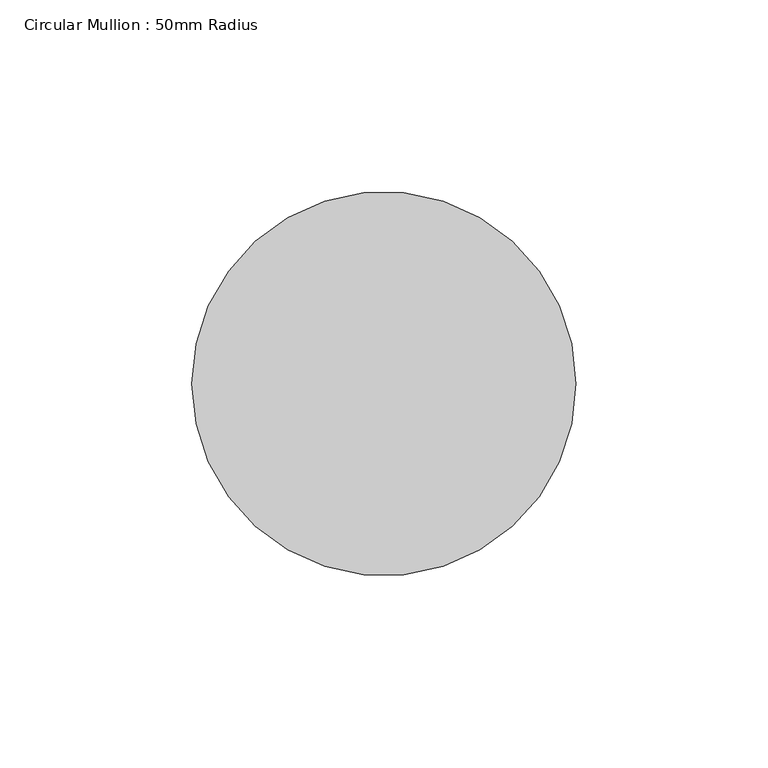
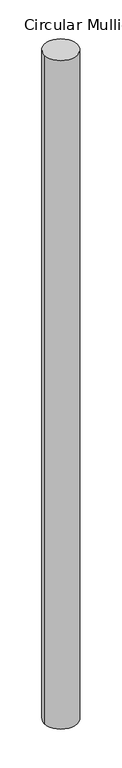
"""IFC4 building model written with IfcOpenShell, lengths in millimetres: member geometry, Circular Mullion : 50mm Radius."""

import ifcopenshell
import ifcopenshell.guid

model = None  # the IFC model being written
_history = None  # IfcOwnerHistory: only IFC2X3 demands one
_inside = {}  # id of a spatial element -> (the spatial element, [elements in it])
_under = {}  # id of a project, library or spatial element -> (it, [spatial elements below it])
_declared = {}  # id of a project -> (the project, [libraries it declares])
_typed = {}  # id of a type object -> (the type object, [elements of that type])
_made_of = {}  # id of a material, layer set ... -> (it, [elements and type objects made of it])


def new_model(schema):
    """Start an empty IFC model of exactly this schema.

    Asked for "IFC4X3", IfcOpenShell would pick the latest addendum, in which some entities
    have other attributes; the version numbers below select the first issue.
    IFC2X3 requires an IfcOwnerHistory on every rooted entity: one is made here for all.
    """
    global model, _history
    if schema == "IFC4X3":
        model = ifcopenshell.file(schema_version=(4, 3, 0, 0))
    else:
        model = ifcopenshell.file(schema=schema)
    _inside.clear()
    _under.clear()
    _declared.clear()
    _typed.clear()
    _made_of.clear()
    _history = None
    if model.schema == "IFC2X3":
        org = make("IfcOrganization", Name="unknown")
        user = make(
            "IfcPersonAndOrganization",
            ThePerson=make("IfcPerson", FamilyName="unknown"),
            TheOrganization=org,
        )
        app = make(
            "IfcApplication",
            ApplicationDeveloper=org,
            Version="unknown",
            ApplicationFullName="unknown",
            ApplicationIdentifier="unknown",
        )
        _history = make(
            "IfcOwnerHistory",
            OwningUser=user,
            OwningApplication=app,
            ChangeAction="ADDED",
            CreationDate=0,
        )
    return model


def make(cls, **values):
    """One entity of the class cls with the attributes given. An attribute that is None is left unset."""
    return model.create_entity(
        cls, **{name: value for name, value in values.items() if value is not None}
    )


def rooted(cls, **values):
    """An entity with a GlobalId (a new one), such as an element, a storey or a relation."""
    return make(cls, GlobalId=ifcopenshell.guid.new(), OwnerHistory=_history, **values)


def si_unit(unit_type, name, prefix=None):
    """IfcSIUnit, for example si_unit("LENGTHUNIT", "METRE", prefix="MILLI")."""
    return make("IfcSIUnit", UnitType=unit_type, Prefix=prefix, Name=name)


def assignment(units):
    """IfcUnitAssignment: the units of a project."""
    return None if units is None else make("IfcUnitAssignment", Units=units)


def point(xyz):
    """IfcCartesianPoint."""
    return None if xyz is None else make("IfcCartesianPoint", Coordinates=xyz)


def direction(xyz):
    """IfcDirection."""
    return None if xyz is None else make("IfcDirection", DirectionRatios=xyz)


def frame(location, z_axis=None, x_axis=None):
    """IfcAxis2Placement3D, a coordinate frame: its origin and axes. An axis left out is left unset."""
    return make(
        "IfcAxis2Placement3D",
        Location=point(location),
        Axis=direction(z_axis),
        RefDirection=direction(x_axis),
    )


def frame_2d(location, x_axis=None):
    """IfcAxis2Placement2D, a coordinate frame in the plane: its origin and x axis."""
    return make(
        "IfcAxis2Placement2D", Location=point(location), RefDirection=direction(x_axis)
    )


def origin():
    """The frame at (0, 0, 0) with its axes left unset."""
    return frame((0.0, 0.0, 0.0))


def place(relative_to, where):
    """IfcLocalPlacement: puts the frame where relative to a parent placement (None: the world)."""
    return make(
        "IfcLocalPlacement", PlacementRelTo=relative_to, RelativePlacement=where
    )


def context(
    kind, dimensions, precision=None, world=None, true_north=None, identifier=None
):
    """IfcGeometricRepresentationContext, for example the 3D "Model" context."""
    return make(
        "IfcGeometricRepresentationContext",
        ContextIdentifier=identifier,
        ContextType=kind,
        CoordinateSpaceDimension=dimensions,
        Precision=precision,
        WorldCoordinateSystem=world,
        TrueNorth=true_north,
    )


def project(units=None, contexts=None):
    """IfcProject with its units and contexts."""
    return rooted(
        "IfcProject",
        Name="project",
        RepresentationContexts=contexts,
        UnitsInContext=assignment(units),
    )


def spatial(cls, under=None, at=None, **own):
    """A site, building, storey or space (cls), placed at a placement, below another one or the project."""
    s = rooted(cls, ObjectPlacement=at, **own)
    if under is not None:
        _under.setdefault(under.id(), (under, []))[1].append(s)
    return s


def circle_curve(where, radius):
    """IfcCircle in the frame where."""
    return make("IfcCircle", Position=where, Radius=radius)


def trimmed(basis, trim1, trim2, sense, master):
    """IfcTrimmedCurve: the piece of a basis curve between two trims."""
    return make(
        "IfcTrimmedCurve",
        BasisCurve=basis,
        Trim1=trim1,
        Trim2=trim2,
        SenseAgreement=sense,
        MasterRepresentation=master,
    )


def segment(curve, same_sense, transition):
    """IfcCompositeCurveSegment."""
    return make(
        "IfcCompositeCurveSegment",
        Transition=transition,
        SameSense=same_sense,
        ParentCurve=curve,
    )


def composite_curve(segments, self_intersect=None):
    """IfcCompositeCurve: segments joined end to end."""
    return make("IfcCompositeCurve", Segments=segments, SelfIntersect=self_intersect)


def outline(outer, holes=None, kind="AREA"):
    """IfcArbitraryClosedProfileDef: a profile drawn as a closed curve; with holes, ...WithVoids."""
    if holes is None:
        return make("IfcArbitraryClosedProfileDef", ProfileType=kind, OuterCurve=outer)
    return make(
        "IfcArbitraryProfileDefWithVoids",
        ProfileType=kind,
        OuterCurve=outer,
        InnerCurves=holes,
    )


def extrude(swept, where, along, depth):
    """IfcExtrudedAreaSolid: the profile swept, set in the frame where, extruded along a direction by depth."""
    return make(
        "IfcExtrudedAreaSolid",
        SweptArea=swept,
        Position=where,
        ExtrudedDirection=direction(along),
        Depth=depth,
    )


def shape(context_of_items, identifier, shape_type, items):
    """IfcShapeRepresentation: the items that make up one representation, for example the "Body"."""
    return make(
        "IfcShapeRepresentation",
        ContextOfItems=context_of_items,
        RepresentationIdentifier=identifier,
        RepresentationType=shape_type,
        Items=items,
    )


def source(mapping_origin, context_of_items, identifier, shape_type, items):
    """IfcRepresentationMap: a shape defined once, which mapped items show again and again."""
    return make(
        "IfcRepresentationMap",
        MappingOrigin=mapping_origin,
        MappedRepresentation=shape(context_of_items, identifier, shape_type, items),
    )


def transform(
    local_origin,
    x_axis=None,
    y_axis=None,
    z_axis=None,
    scale=None,
    scale2=None,
    scale3=None,
    uniform=True,
):
    """IfcCartesianTransformationOperator3D, or its non-uniform kind. x_axis, y_axis, z_axis: its Axis1, 2, 3."""
    if uniform:
        return make(
            "IfcCartesianTransformationOperator3D",
            Axis1=direction(x_axis),
            Axis2=direction(y_axis),
            LocalOrigin=point(local_origin),
            Scale=scale,
            Axis3=direction(z_axis),
        )
    return make(
        "IfcCartesianTransformationOperator3DnonUniform",
        Axis1=direction(x_axis),
        Axis2=direction(y_axis),
        LocalOrigin=point(local_origin),
        Scale=scale,
        Axis3=direction(z_axis),
        Scale2=scale2,
        Scale3=scale3,
    )


def mapped(mapping_source, mapping_target):
    """IfcMappedItem: shows the shape of a source again, moved by a transform."""
    return make(
        "IfcMappedItem", MappingSource=mapping_source, MappingTarget=mapping_target
    )


def made_of(thing, what):
    """Note that an element or type object is made of a material, layer set ...; save() writes the relation."""
    if what is not None:
        _made_of.setdefault(what.id(), (what, []))[1].append(thing)
    return thing


def element(
    cls,
    number,
    at=None,
    inside=None,
    cuts=None,
    type_object=None,
    material=None,
    context=None,
    identifier="Body",
    shape_type=None,
    held_by="IfcProductDefinitionShape",
    body=None,
    shapes=None,
    **own,
):
    """One element of the class cls, such as IfcWall. Its Tag is "e" and its number.

    at: its placement. inside: the storey or other place that contains it. cuts: it is an
    opening in that element (IfcRelVoidsElement). A single representation is given by context,
    identifier, shape_type and body (its items); several are given by shapes. held_by: the class
    of the entity that holds the representations. save() writes the other relations.
    """
    e = rooted(cls, Tag="e%d" % number, ObjectPlacement=at, **own)
    if body is not None:
        shapes = [shape(context, identifier, shape_type, body)]
    if shapes is not None:
        e.Representation = make(held_by, Representations=shapes)
    if inside is not None:
        _inside.setdefault(inside.id(), (inside, []))[1].append(e)
    if cuts is not None:
        rooted(
            "IfcRelVoidsElement", RelatingBuildingElement=cuts, RelatedOpeningElement=e
        )
    if type_object is not None:
        _typed.setdefault(type_object.id(), (type_object, []))[1].append(e)
    return made_of(e, material)


def aggregate(whole, parts):
    """IfcRelAggregates: a whole, such as a stair, and the parts it consists of."""
    return rooted("IfcRelAggregates", RelatingObject=whole, RelatedObjects=parts)


def save(model, path):
    """Write the relations noted so far, then the file.

    IfcRelAggregates (storeys below a building ...), IfcRelContainedInSpatialStructure (elements
    in a storey), IfcRelDefinesByType, IfcRelAssociatesMaterial and IfcRelDeclares: one each for
    every whole, place, type object, material and project.
    """
    for whole, parts in _under.values():
        aggregate(whole, parts)
    for where, things in _inside.values():
        rooted(
            "IfcRelContainedInSpatialStructure",
            RelatedElements=things,
            RelatingStructure=where,
        )
    for kind, things in _typed.values():
        rooted("IfcRelDefinesByType", RelatedObjects=things, RelatingType=kind)
    for what, things in _made_of.values():
        rooted("IfcRelAssociatesMaterial", RelatedObjects=things, RelatingMaterial=what)
    for by, libraries in _declared.values():
        rooted("IfcRelDeclares", RelatingContext=by, RelatedDefinitions=libraries)
    model.write(path)


def circular_mullion_50mm_radius_329bae3a(model_context):
    return source(origin(), model_context, "Body", "SweptSolid", [
        extrude(outline(composite_curve([segment(trimmed(circle_curve(frame_2d((-50.0, 0.0)), 50.0), [point((0.0, 0.0))], [point((-100.0, 0.0))], False, "CARTESIAN"), True, "CONTINUOUS"), segment(trimmed(circle_curve(frame_2d((-50.0, 0.0)), 50.0), [point((-100.0, 0.0))], [point((0.0, 0.0))], False, "CARTESIAN"), True, "CONTINUOUS")], self_intersect=False)), frame((0.0, 0.0, -2152.4790122), z_axis=(0.0, 0.0, 1.0), x_axis=(1.0, 0.0, 0.0)), (0.0, 0.0, 1.0), 2152.4790122),
    ])


if __name__ == "__main__":
    model = new_model("IFC4")
    model_context = context("Model", 3, world=origin())
    ifc_project = project(units=[si_unit("LENGTHUNIT", "METRE", prefix="MILLI")], contexts=[model_context])
    site = spatial("IfcSite", under=ifc_project)
    building = spatial("IfcBuilding", under=site)
    placement = place(None, origin())
    circular_mullion_50mm_radius_shape = circular_mullion_50mm_radius_329bae3a(model_context)
    element("IfcMember", 1, ObjectType="Circular Mullion : 50mm Radius", at=placement, inside=building, context=model_context, shape_type="MappedRepresentation", body=[
        mapped(circular_mullion_50mm_radius_shape, transform((0.0, 0.0, 0.0), x_axis=(1.0, 0.0, 0.0), y_axis=(0.0, 1.0, 0.0), z_axis=(0.0, 0.0, 1.0))),
    ])
    save(model, "model.ifc")

# Revit data of these elements
# Type "Circular Mullion : 50mm Radius"
#   built-in parameter 1007350 = 0.164042 (stored number, unit not read)
# Element 1 (IfcMember, "Circular Mullion : 50mm Radius")
#   Materials on its faces: "Aluminium"
# Materials
#   "Aluminium": class "Metal", colour RGB 247 247 247, transparency 0, Description = "Aluminium 6061", Cost = 0
